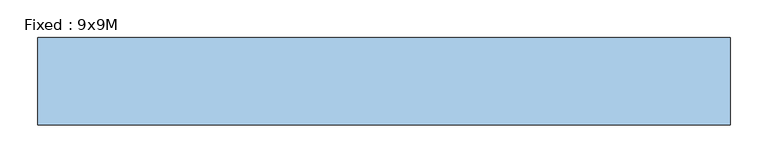
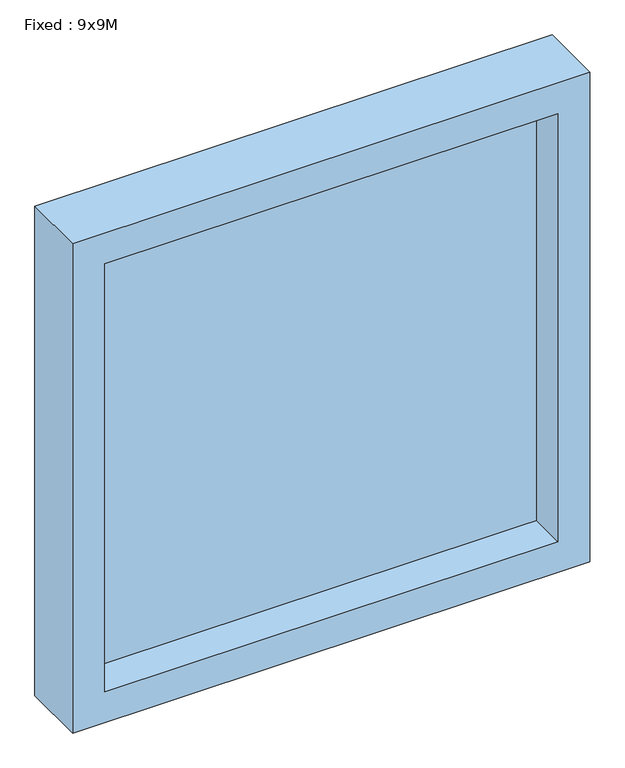
"""IFC4 building model written with IfcOpenShell, lengths in millimetres: window geometry, Fixed : 9x9M."""

from ifc_helpers import new_model, si_unit, frame, origin, place, context, project, spatial, polyline, outline, extrude, source, transform, mapped, element, save


def fixed_9x9m_da96294a(model_context):
    return source(origin(), model_context, "Body", "SweptSolid", [
        extrude(outline(polyline([(1712.0, 456.0), (1712.0, -456.0), (800.0, -456.0), (800.0, 456.0), (1712.0, 456.0)]), holes=[polyline([(857.0, 399.0), (857.0, -399.0), (1655.0, -399.0), (1655.0, 399.0), (857.0, 399.0)])]), frame((0.0, 69.0, 0.0), z_axis=(0.0, 1.0, 0.0), x_axis=(0.0, 0.0, 1.0)), (0.0, 0.0, 1.0), 115.0),
        extrude(outline(polyline([(-399.0, 162.0), (399.0, 162.0), (399.0, 134.0), (-399.0, 134.0), (-399.0, 162.0)])), frame((0.0, 0.0, 857.0), z_axis=(0.0, 0.0, 1.0), x_axis=(1.0, 0.0, 0.0)), (0.0, 0.0, 1.0), 798.0),
    ])


if __name__ == "__main__":
    model = new_model("IFC4")
    model_context = context("Model", 3, world=origin())
    ifc_project = project(units=[si_unit("LENGTHUNIT", "METRE", prefix="MILLI")], contexts=[model_context])
    site = spatial("IfcSite", under=ifc_project)
    building = spatial("IfcBuilding", under=site)
    placement = place(None, origin())
    fixed_9x9m_shape = fixed_9x9m_da96294a(model_context)
    element("IfcWindow", 1, ObjectType="Fixed : 9x9M", at=placement, inside=building, context=model_context, shape_type="MappedRepresentation", body=[
        mapped(fixed_9x9m_shape, transform((0.0, 0.0, 0.0), x_axis=(1.0, 0.0, 0.0), y_axis=(0.0, 1.0, 0.0), z_axis=(0.0, 0.0, 1.0))),
    ])
    save(model, "model.ifc")

# Revit data of these elements
# Type "Fixed : 9x9M"
#   Type Mark = "46"
#   Creator Organization [instance default] = "© Danish Educational Content"
#   Creator Name [instance default] = "© Erik Falck Jørgensen"
#   Creator Build [instance default] = "2017.0801.0"
#   Analytic Construction = "<None>"
#   length#5 = -22 mm
#   length#4 = -50 mm
#   length#3 = 100 mm
#   length#2 = 57 mm
#   length#1 = 0 mm
#   Seal Width = 12 mm
#   Rough Width = 912 mm
#   Rough Height = 912 mm
#   Rebate Depth = 50 mm
#   Height = 888 mm
#   Glass Thickness = 28 mm
#   Exterior Direction [instance default] = 0.00°
#   Default Sill Height = 800 mm
#   Width = 888 mm
#   Case Width = 45 mm
#   Case Depth = 115 mm
#   Sealing = no
#   Wall Closure = 1
#   Above Cutplane [instance default] = no
#   Wall Surface = none
#   Sill Plate = none
#   Glass = none
#   Embrasure = none
#   Case/Transom = none
#   Assembly Code = ""
# Element 1 (IfcWindow, "Fixed : 9x9M")
#   Materials on its faces: "Default Frame/Mullion (Interior/Exterior)", "Glass"
# Materials
#   "Default Frame/Mullion (Interior/Exterior)": class "Generic", colour RGB 205 205 205, transparency 0, Description = "Udefineret karm/ramme materiale", Cost = 0
#   "Glass": class "Glass", colour RGB 180 200 255, transparency 0.75, Description = "Generisk glas", Cost = 0
